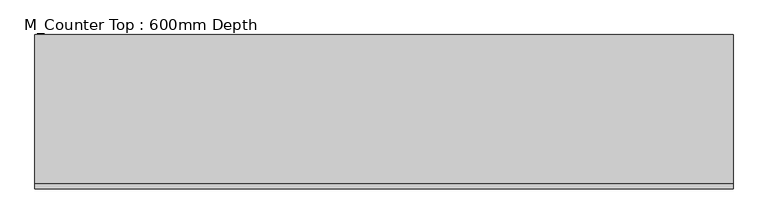
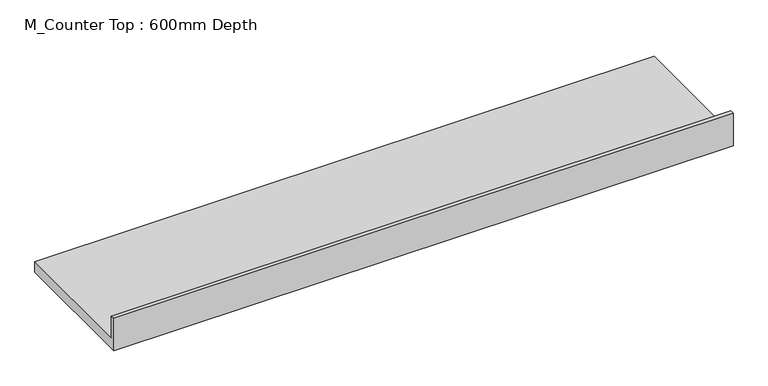
"""IFC4 building model written with IfcOpenShell, lengths in millimetres: furniture geometry, M_Counter Top : 600mm Depth."""

from ifc_helpers import new_model, si_unit, frame, origin, place, context, project, spatial, polyline, outline, extrude, source, transform, mapped, element, save


def m_counter_top_600mm_depth_535bf1f1(model_context):
    return source(origin(), model_context, "Body", "SweptSolid", [
        extrude(outline(polyline([(0.0, 1016.0), (19.05, 1016.0), (19.05, 914.4), (609.6, 914.4), (609.6, 863.6), (0.0, 863.6), (0.0, 1016.0)])), frame((-1200.4622951, 0.0, 0.0), z_axis=(1.0, 0.0, 0.0), x_axis=(0.0, 1.0, 0.0)), (0.0, 0.0, 1.0), 2756.3233509),
    ])


if __name__ == "__main__":
    model = new_model("IFC4")
    model_context = context("Model", 3, world=origin())
    ifc_project = project(units=[si_unit("LENGTHUNIT", "METRE", prefix="MILLI")], contexts=[model_context])
    site = spatial("IfcSite", under=ifc_project)
    building = spatial("IfcBuilding", under=site)
    placement = place(None, origin())
    m_counter_top_600mm_depth_shape = m_counter_top_600mm_depth_535bf1f1(model_context)
    element("IfcFurniture", 1, ObjectType="M_Counter Top : 600mm Depth", at=placement, inside=building, context=model_context, shape_type="MappedRepresentation", body=[
        mapped(m_counter_top_600mm_depth_shape, transform((0.0, 0.0, 0.0), x_axis=(1.0, 0.0, 0.0), y_axis=(0.0, 1.0, 0.0), z_axis=(0.0, 0.0, 1.0))),
    ])
    save(model, "model.ifc")

# Revit data of these elements
# Type "M_Counter Top : 600mm Depth"
#   Counter Thickness = 0' - 2"
#   Depth = 2' - 0"
#   Height = 3' - 0"
#   Length [instance default] = 8' - 2.4252"
#   Counter Top Material = MAX HEIGHT OF COUNTERTOP 34"
# Element 1 (IfcFurniture, "M_Counter Top : 600mm Depth")
#   Length = 9' - 0.51667"
#   Materials on its faces: "MAX HEIGHT OF COUNTERTOP 34\""
# Materials
#   "MAX HEIGHT OF COUNTERTOP 34\"": class "Wood", colour RGB 226 177 128, transparency 0, Cost = 0
